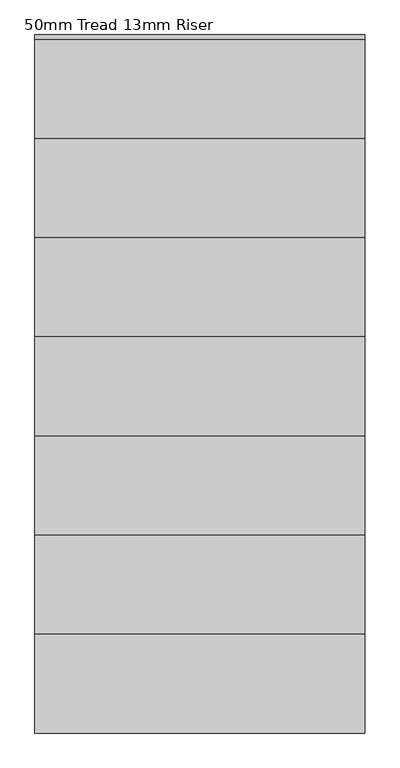
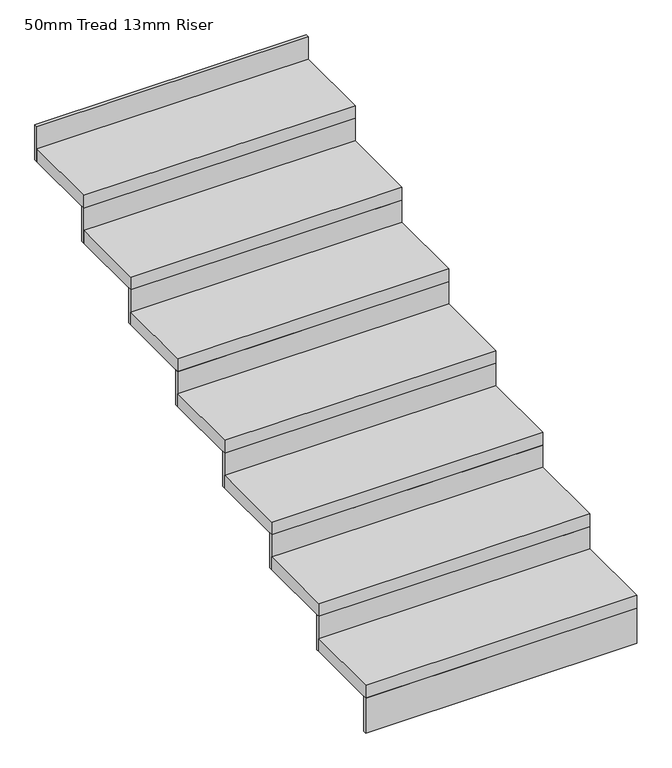
"""IFC4 building model written with IfcOpenShell, lengths in millimetres: stair flight geometry, 50mm Tread 13mm Riser."""

from ifc_helpers import new_model, si_unit, frame, origin, place, context, project, spatial, polyline, outline, extrude, source, transform, mapped, element, save


def stair_flight_50mm_tread_13mm_riser_8a60ed0c(model_context):
    return source(origin(), model_context, "Body", "SweptSolid", [
        extrude(outline(polyline([(22749.836337, -2888.024372), (22749.836337, -2900.524372), (21749.836337, -2900.524372), (21749.836337, -2888.024372), (22749.836337, -2888.024372)])), frame((0.0, 0.0, 1859.0909091), z_axis=(0.0, 0.0, 1.0), x_axis=(1.0, 0.0, 0.0)), (0.0, 0.0, 1.0), 136.3636364),
        extrude(outline(polyline([(21749.836337, -2600.524372), (22749.836337, -2600.524372), (22749.836337, -2900.524372), (21749.836337, -2900.524372), (21749.836337, -2600.524372)])), frame((0.0, 0.0, 1995.4545455), z_axis=(0.0, 0.0, 1.0), x_axis=(1.0, 0.0, 0.0)), (0.0, 0.0, 1.0), 50.0),
        extrude(outline(polyline([(22749.836337, -2588.024372), (22749.836337, -2600.524372), (21749.836337, -2600.524372), (21749.836337, -2588.024372), (22749.836337, -2588.024372)])), frame((0.0, 0.0, 1995.4545455), z_axis=(0.0, 0.0, 1.0), x_axis=(1.0, 0.0, 0.0)), (0.0, 0.0, 1.0), 136.3636364),
        extrude(outline(polyline([(21749.836337, -2300.524372), (22749.836337, -2300.524372), (22749.836337, -2600.524372), (21749.836337, -2600.524372), (21749.836337, -2300.524372)])), frame((0.0, 0.0, 2131.8181818), z_axis=(0.0, 0.0, 1.0), x_axis=(1.0, 0.0, 0.0)), (0.0, 0.0, 1.0), 50.0),
        extrude(outline(polyline([(22749.836337, -2288.024372), (22749.836337, -2300.524372), (21749.836337, -2300.524372), (21749.836337, -2288.024372), (22749.836337, -2288.024372)])), frame((0.0, 0.0, 2131.8181818), z_axis=(0.0, 0.0, 1.0), x_axis=(1.0, 0.0, 0.0)), (0.0, 0.0, 1.0), 136.3636364),
        extrude(outline(polyline([(21749.836337, -2000.524372), (22749.836337, -2000.524372), (22749.836337, -2300.524372), (21749.836337, -2300.524372), (21749.836337, -2000.524372)])), frame((0.0, 0.0, 2268.1818182), z_axis=(0.0, 0.0, 1.0), x_axis=(1.0, 0.0, 0.0)), (0.0, 0.0, 1.0), 50.0),
        extrude(outline(polyline([(22749.836337, -1988.024372), (22749.836337, -2000.524372), (21749.836337, -2000.524372), (21749.836337, -1988.024372), (22749.836337, -1988.024372)])), frame((0.0, 0.0, 2268.1818182), z_axis=(0.0, 0.0, 1.0), x_axis=(1.0, 0.0, 0.0)), (0.0, 0.0, 1.0), 136.3636364),
        extrude(outline(polyline([(21749.836337, -1700.524372), (22749.836337, -1700.524372), (22749.836337, -2000.524372), (21749.836337, -2000.524372), (21749.836337, -1700.524372)])), frame((0.0, 0.0, 2404.5454545), z_axis=(0.0, 0.0, 1.0), x_axis=(1.0, 0.0, 0.0)), (0.0, 0.0, 1.0), 50.0),
        extrude(outline(polyline([(22749.836337, -1688.024372), (22749.836337, -1700.524372), (21749.836337, -1700.524372), (21749.836337, -1688.024372), (22749.836337, -1688.024372)])), frame((0.0, 0.0, 2404.5454545), z_axis=(0.0, 0.0, 1.0), x_axis=(1.0, 0.0, 0.0)), (0.0, 0.0, 1.0), 136.3636364),
        extrude(outline(polyline([(21749.836337, -1400.524372), (22749.836337, -1400.524372), (22749.836337, -1700.524372), (21749.836337, -1700.524372), (21749.836337, -1400.524372)])), frame((0.0, 0.0, 2540.9090909), z_axis=(0.0, 0.0, 1.0), x_axis=(1.0, 0.0, 0.0)), (0.0, 0.0, 1.0), 50.0),
        extrude(outline(polyline([(22749.836337, -1388.024372), (22749.836337, -1400.524372), (21749.836337, -1400.524372), (21749.836337, -1388.024372), (22749.836337, -1388.024372)])), frame((0.0, 0.0, 2540.9090909), z_axis=(0.0, 0.0, 1.0), x_axis=(1.0, 0.0, 0.0)), (0.0, 0.0, 1.0), 136.3636364),
        extrude(outline(polyline([(21749.836337, -1100.524372), (22749.836337, -1100.524372), (22749.836337, -1400.524372), (21749.836337, -1400.524372), (21749.836337, -1100.524372)])), frame((0.0, 0.0, 2677.2727273), z_axis=(0.0, 0.0, 1.0), x_axis=(1.0, 0.0, 0.0)), (0.0, 0.0, 1.0), 50.0),
        extrude(outline(polyline([(22749.836337, -1088.024372), (22749.836337, -1100.524372), (21749.836337, -1100.524372), (21749.836337, -1088.024372), (22749.836337, -1088.024372)])), frame((0.0, 0.0, 2677.2727273), z_axis=(0.0, 0.0, 1.0), x_axis=(1.0, 0.0, 0.0)), (0.0, 0.0, 1.0), 136.3636364),
        extrude(outline(polyline([(21749.836337, -800.524372), (22749.836337, -800.524372), (22749.836337, -1100.524372), (21749.836337, -1100.524372), (21749.836337, -800.524372)])), frame((0.0, 0.0, 2813.6363636), z_axis=(0.0, 0.0, 1.0), x_axis=(1.0, 0.0, 0.0)), (0.0, 0.0, 1.0), 50.0),
        extrude(outline(polyline([(22749.836337, -788.024372), (22749.836337, -800.524372), (21749.836337, -800.524372), (21749.836337, -788.024372), (22749.836337, -788.024372)])), frame((0.0, 0.0, 2813.6363636), z_axis=(0.0, 0.0, 1.0), x_axis=(1.0, 0.0, 0.0)), (0.0, 0.0, 1.0), 136.3636364),
    ])


if __name__ == "__main__":
    model = new_model("IFC4")
    model_context = context("Model", 3, world=origin())
    ifc_project = project(units=[si_unit("LENGTHUNIT", "METRE", prefix="MILLI")], contexts=[model_context])
    site = spatial("IfcSite", under=ifc_project)
    building = spatial("IfcBuilding", under=site)
    placement = place(None, origin())
    stair_flight_50mm_tread_13mm_riser_shape = stair_flight_50mm_tread_13mm_riser_8a60ed0c(model_context)
    element("IfcStairFlight", 1, ObjectType="50mm Tread 13mm Riser", at=placement, inside=building, context=model_context, shape_type="MappedRepresentation", body=[
        mapped(stair_flight_50mm_tread_13mm_riser_shape, transform((0.0, 0.0, 0.0), x_axis=(1.0, 0.0, 0.0), y_axis=(0.0, 1.0, 0.0), z_axis=(0.0, 0.0, 1.0))),
    ])
    save(model, "model.ifc")
